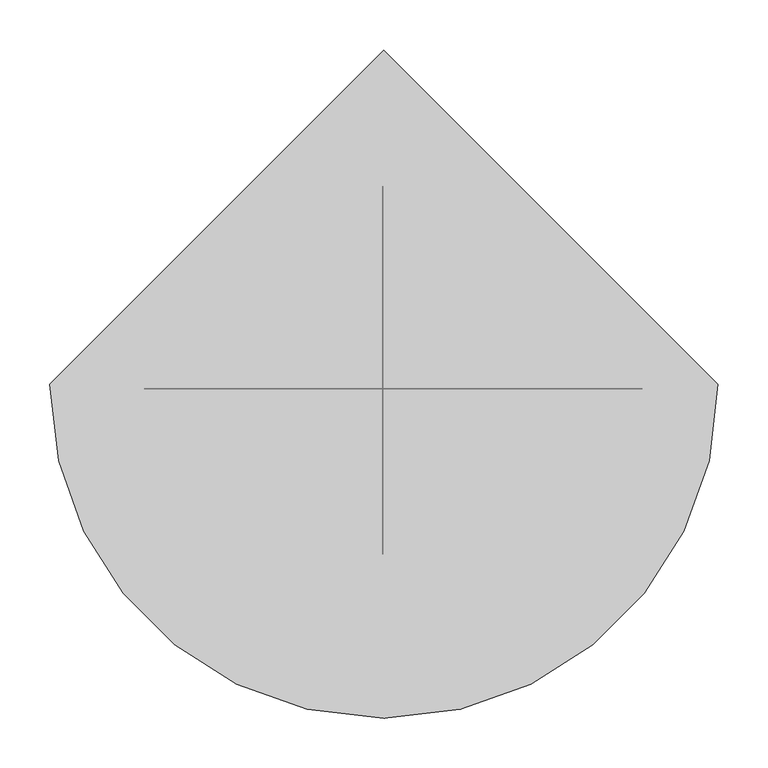
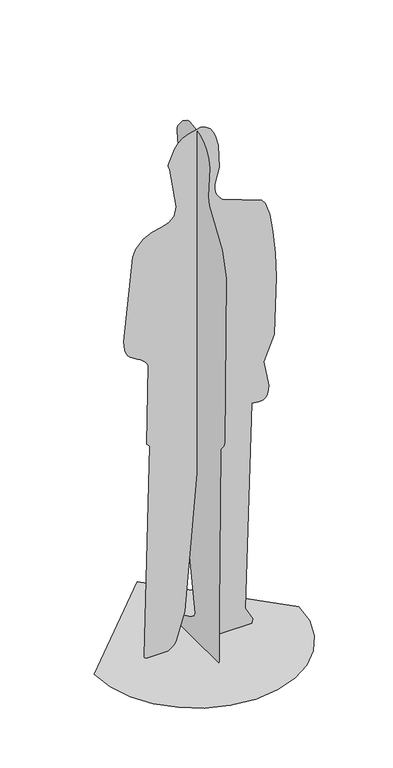
"""IFC4 building model written with IfcOpenShell, lengths in millimetres: proxy geometry, dwayne 23733 : dwayne 23733."""

import ifcopenshell
import ifcopenshell.guid

model = None  # the IFC model being written
_history = None  # IfcOwnerHistory: only IFC2X3 demands one
_inside = {}  # id of a spatial element -> (the spatial element, [elements in it])
_under = {}  # id of a project, library or spatial element -> (it, [spatial elements below it])
_declared = {}  # id of a project -> (the project, [libraries it declares])
_typed = {}  # id of a type object -> (the type object, [elements of that type])
_made_of = {}  # id of a material, layer set ... -> (it, [elements and type objects made of it])


def new_model(schema):
    """Start an empty IFC model of exactly this schema.

    Asked for "IFC4X3", IfcOpenShell would pick the latest addendum, in which some entities
    have other attributes; the version numbers below select the first issue.
    IFC2X3 requires an IfcOwnerHistory on every rooted entity: one is made here for all.
    """
    global model, _history
    if schema == "IFC4X3":
        model = ifcopenshell.file(schema_version=(4, 3, 0, 0))
    else:
        model = ifcopenshell.file(schema=schema)
    _inside.clear()
    _under.clear()
    _declared.clear()
    _typed.clear()
    _made_of.clear()
    _history = None
    if model.schema == "IFC2X3":
        org = make("IfcOrganization", Name="unknown")
        user = make(
            "IfcPersonAndOrganization",
            ThePerson=make("IfcPerson", FamilyName="unknown"),
            TheOrganization=org,
        )
        app = make(
            "IfcApplication",
            ApplicationDeveloper=org,
            Version="unknown",
            ApplicationFullName="unknown",
            ApplicationIdentifier="unknown",
        )
        _history = make(
            "IfcOwnerHistory",
            OwningUser=user,
            OwningApplication=app,
            ChangeAction="ADDED",
            CreationDate=0,
        )
    return model


def make(cls, **values):
    """One entity of the class cls with the attributes given. An attribute that is None is left unset."""
    return model.create_entity(
        cls, **{name: value for name, value in values.items() if value is not None}
    )


def rooted(cls, **values):
    """An entity with a GlobalId (a new one), such as an element, a storey or a relation."""
    return make(cls, GlobalId=ifcopenshell.guid.new(), OwnerHistory=_history, **values)


def si_unit(unit_type, name, prefix=None):
    """IfcSIUnit, for example si_unit("LENGTHUNIT", "METRE", prefix="MILLI")."""
    return make("IfcSIUnit", UnitType=unit_type, Prefix=prefix, Name=name)


def assignment(units):
    """IfcUnitAssignment: the units of a project."""
    return None if units is None else make("IfcUnitAssignment", Units=units)


def point(xyz):
    """IfcCartesianPoint."""
    return None if xyz is None else make("IfcCartesianPoint", Coordinates=xyz)


def direction(xyz):
    """IfcDirection."""
    return None if xyz is None else make("IfcDirection", DirectionRatios=xyz)


def frame(location, z_axis=None, x_axis=None):
    """IfcAxis2Placement3D, a coordinate frame: its origin and axes. An axis left out is left unset."""
    return make(
        "IfcAxis2Placement3D",
        Location=point(location),
        Axis=direction(z_axis),
        RefDirection=direction(x_axis),
    )


def origin():
    """The frame at (0, 0, 0) with its axes left unset."""
    return frame((0.0, 0.0, 0.0))


def place(relative_to, where):
    """IfcLocalPlacement: puts the frame where relative to a parent placement (None: the world)."""
    return make(
        "IfcLocalPlacement", PlacementRelTo=relative_to, RelativePlacement=where
    )


def context(
    kind, dimensions, precision=None, world=None, true_north=None, identifier=None
):
    """IfcGeometricRepresentationContext, for example the 3D "Model" context."""
    return make(
        "IfcGeometricRepresentationContext",
        ContextIdentifier=identifier,
        ContextType=kind,
        CoordinateSpaceDimension=dimensions,
        Precision=precision,
        WorldCoordinateSystem=world,
        TrueNorth=true_north,
    )


def project(units=None, contexts=None):
    """IfcProject with its units and contexts."""
    return rooted(
        "IfcProject",
        Name="project",
        RepresentationContexts=contexts,
        UnitsInContext=assignment(units),
    )


def spatial(cls, under=None, at=None, **own):
    """A site, building, storey or space (cls), placed at a placement, below another one or the project."""
    s = rooted(cls, ObjectPlacement=at, **own)
    if under is not None:
        _under.setdefault(under.id(), (under, []))[1].append(s)
    return s


def point_list(points):
    """IfcCartesianPointList2D or 3D."""
    cls = (
        "IfcCartesianPointList2D" if len(points[0]) == 2 else "IfcCartesianPointList3D"
    )
    return make(cls, CoordList=points)


def triangles(points, corners, closed=None, point_numbers=None):
    """IfcTriangulatedFaceSet: each triangle names its three corners, points numbered from 1."""
    return make(
        "IfcTriangulatedFaceSet",
        Coordinates=point_list(points),
        Closed=closed,
        CoordIndex=corners,
        PnIndex=point_numbers,
    )


def shape(context_of_items, identifier, shape_type, items):
    """IfcShapeRepresentation: the items that make up one representation, for example the "Body"."""
    return make(
        "IfcShapeRepresentation",
        ContextOfItems=context_of_items,
        RepresentationIdentifier=identifier,
        RepresentationType=shape_type,
        Items=items,
    )


def source(mapping_origin, context_of_items, identifier, shape_type, items):
    """IfcRepresentationMap: a shape defined once, which mapped items show again and again."""
    return make(
        "IfcRepresentationMap",
        MappingOrigin=mapping_origin,
        MappedRepresentation=shape(context_of_items, identifier, shape_type, items),
    )


def transform(
    local_origin,
    x_axis=None,
    y_axis=None,
    z_axis=None,
    scale=None,
    scale2=None,
    scale3=None,
    uniform=True,
):
    """IfcCartesianTransformationOperator3D, or its non-uniform kind. x_axis, y_axis, z_axis: its Axis1, 2, 3."""
    if uniform:
        return make(
            "IfcCartesianTransformationOperator3D",
            Axis1=direction(x_axis),
            Axis2=direction(y_axis),
            LocalOrigin=point(local_origin),
            Scale=scale,
            Axis3=direction(z_axis),
        )
    return make(
        "IfcCartesianTransformationOperator3DnonUniform",
        Axis1=direction(x_axis),
        Axis2=direction(y_axis),
        LocalOrigin=point(local_origin),
        Scale=scale,
        Axis3=direction(z_axis),
        Scale2=scale2,
        Scale3=scale3,
    )


def mapped(mapping_source, mapping_target):
    """IfcMappedItem: shows the shape of a source again, moved by a transform."""
    return make(
        "IfcMappedItem", MappingSource=mapping_source, MappingTarget=mapping_target
    )


def made_of(thing, what):
    """Note that an element or type object is made of a material, layer set ...; save() writes the relation."""
    if what is not None:
        _made_of.setdefault(what.id(), (what, []))[1].append(thing)
    return thing


def element(
    cls,
    number,
    at=None,
    inside=None,
    cuts=None,
    type_object=None,
    material=None,
    context=None,
    identifier="Body",
    shape_type=None,
    held_by="IfcProductDefinitionShape",
    body=None,
    shapes=None,
    **own,
):
    """One element of the class cls, such as IfcWall. Its Tag is "e" and its number.

    at: its placement. inside: the storey or other place that contains it. cuts: it is an
    opening in that element (IfcRelVoidsElement). A single representation is given by context,
    identifier, shape_type and body (its items); several are given by shapes. held_by: the class
    of the entity that holds the representations. save() writes the other relations.
    """
    e = rooted(cls, Tag="e%d" % number, ObjectPlacement=at, **own)
    if body is not None:
        shapes = [shape(context, identifier, shape_type, body)]
    if shapes is not None:
        e.Representation = make(held_by, Representations=shapes)
    if inside is not None:
        _inside.setdefault(inside.id(), (inside, []))[1].append(e)
    if cuts is not None:
        rooted(
            "IfcRelVoidsElement", RelatingBuildingElement=cuts, RelatedOpeningElement=e
        )
    if type_object is not None:
        _typed.setdefault(type_object.id(), (type_object, []))[1].append(e)
    return made_of(e, material)


def aggregate(whole, parts):
    """IfcRelAggregates: a whole, such as a stair, and the parts it consists of."""
    return rooted("IfcRelAggregates", RelatingObject=whole, RelatedObjects=parts)


def save(model, path):
    """Write the relations noted so far, then the file.

    IfcRelAggregates (storeys below a building ...), IfcRelContainedInSpatialStructure (elements
    in a storey), IfcRelDefinesByType, IfcRelAssociatesMaterial and IfcRelDeclares: one each for
    every whole, place, type object, material and project.
    """
    for whole, parts in _under.values():
        aggregate(whole, parts)
    for where, things in _inside.values():
        rooted(
            "IfcRelContainedInSpatialStructure",
            RelatedElements=things,
            RelatingStructure=where,
        )
    for kind, things in _typed.values():
        rooted("IfcRelDefinesByType", RelatedObjects=things, RelatingType=kind)
    for what, things in _made_of.values():
        rooted("IfcRelAssociatesMaterial", RelatedObjects=things, RelatingMaterial=what)
    for by, libraries in _declared.values():
        rooted("IfcRelDeclares", RelatingContext=by, RelatedDefinitions=libraries)
    model.write(path)


def entourage_8da15c99(model_context):
    return source(origin(), model_context, "Body", "Tessellation", [
        triangles([(-180.7520848, -4.45e-05, 5.61e-05), (-184.2428783, -8.8e-06, 2.7953159), (-186.1722845, 1.66e-05, 5.8375037), (-186.8317464, 3.35e-05, 9.1275741), (-168.2847317, 8.5e-06, 733.0655743), (-173.8813923, 8.5e-06, 735.2245268), (-177.6699692, 8.1e-06, 740.933626), (-174.1986513, -8.1e-06, 1013.6688681), (-179.5913999, -8.8e-06, 1024.1657564), (-188.0396306, -9.6e-06, 1032.776568), (-198.5268356, -9.9e-06, 1040.1131842), (-210.0364347, -1.03e-05, 1046.7870501), (-221.5521744, -1.07e-05, 1053.4099016), (-232.0573471, -1.1e-05, 1060.5935474), (-240.5355178, -1.14e-05, 1068.9495054), (-245.9520113, -1.21e-05, 1078.9886456), (-249.7388442, -1.29e-05, 1091.9828379), (-252.1553936, -1.4e-05, 1106.9305447), (-253.4609098, -1.47e-05, 1122.8302282), (-224.2189811, -3.16e-05, 1405.0555161), (-213.7950534, -3.31e-05, 1430.2028183), (-189.1320784, -3.46e-05, 1456.0851048), (-160.6250248, -3.53e-05, 1468.8744404), (-131.9230613, -3.57e-05, 1475.6387077), (-106.6753564, -3.64e-05, 1483.4444813), (-88.5310787, -3.71e-05, 1499.3602249), (-81.1393152, -3.9e-05, 1530.4525131), (-102.9420995, -4.71e-05, 1666.4706642), (-107.9473082, -4.78e-05, 1679.2661041), (-108.147514, -4.82e-05, 1680.5750359), (-107.9848786, -4.82e-05, 1682.7597862), (-107.5268942, -4.82e-05, 1685.5199375), (-106.8410076, -4.86e-05, 1688.5562347), (-86.6409597, -5.11e-05, 1733.0913071), (-74.2774747, -5.19e-05, 1747.7193386), (-59.5121968, -5.26e-05, 1759.6604702), (-42.3631437, -5.33e-05, 1768.778809), (-0.985526, -5.37e-05, 1778.0000484), (15.8808848, -5.33e-05, 1772.5538692), (29.1619713, -5.26e-05, 1761.5650051), (39.2640596, -5.19e-05, 1747.0972836), (46.5934905, -5.08e-05, 1731.2151134), (56.0091948, -4.89e-05, 1695.7216404), (59.1639804, -4.41e-05, 1618.2096565), (44.4858611, -4.12e-05, 1564.728764), (44.3096955, -4.05e-05, 1551.1871487), (46.5533085, -3.94e-05, 1537.928801), (51.2886617, -3.86e-05, 1525.4368309), (58.5876893, -3.83e-05, 1514.1934765), (68.5223573, -3.75e-05, 1504.6817024), (198.4031332, -3.46e-05, 1454.5817081), (210.7096676, -3.38e-05, 1440.8303673), (224.9007164, -3.13e-05, 1397.8456364), (235.5370584, -2.72e-05, 1333.6076969), (242.7581838, -2.28e-05, 1256.1539944), (246.7033826, -1.77e-05, 1173.5217562), (240.2782843, -5.9e-06, 974.9295902), (206.0815162, -1.1e-06, 891.6227566), (221.1963095, 4e-06, 805.6638319), (220.4651949, 5.1e-06, 788.6204681), (214.9949983, 6.3e-06, 771.8049974), (210.3553288, 6.6e-06, 765.7305136), (204.1669347, 6.6e-06, 762.0923635), (196.896103, 7e-06, 760.3986443), (189.0091026, 7e-06, 760.1578159), (180.9722385, 7e-06, 760.8779028), (173.2516706, 6.6e-06, 762.0673651), (166.3136674, 6.6e-06, 763.2343723), (144.8011997, 4.49e-05, 59.4753214), (168.6276432, 4.74e-05, 15.3365923), (166.1986854, -4.45e-05, 5.61e-05), (66.1332453, -4.45e-05, 5.61e-05), (49.8425291, -1.03e-05, 3.9765614), (39.0246438, 1.36e-05, 14.0353079), (32.5983191, 2.91e-05, 28.3297275), (-2.744106, 9.2e-06, 720.0463108), (-54.0725352, 1.03e-05, 117.9433913), (-81.3720589, -2.13e-05, 28.0047586), (-85.5237496, -2.69e-05, 19.9172799), (-91.2434313, -3.27e-05, 12.5691251), (-99.2452049, -3.86e-05, 5.9378921), (-110.2432618, -4.45e-05, 5.61e-05), (-13.8237486, -127.6719491, 9.9621213), (-13.8238053, -127.261836, 182.0843436), (-13.8237894, -135.2636459, 744.8700136), (-13.8237894, -136.4150655, 748.3464729), (-13.8237894, -139.3955521, 752.5740492), (-13.8237894, -143.4944844, 757.5063063), (-13.8237894, -148.0011678, 763.0967354), (-13.8237894, -152.2050719, 769.2988277), (-13.8237872, -155.3954567, 776.0660746), (-13.8237872, -156.8617189, 783.3521124), (-13.8237701, -165.9465932, 1358.6144554), (-13.8237679, -143.2744033, 1442.0936623), (-13.8237656, -71.1145909, 1552.8595757), (-13.8237656, -64.3402088, 1580.52155), (-13.8237622, -73.5344423, 1684.7962898), (-13.823761, -67.2131621, 1712.2171452), (-13.823761, -55.2412548, 1734.9080566), (-13.823761, -37.926044, 1752.7547871), (-13.823761, -15.5748862, 1765.6435352), (-13.823761, 11.5049153, 1773.4603546), (-13.823761, 43.0060141, 1776.0911533), (-13.823761, 55.0860544, 1772.9175098), (-13.8237622, 79.7039013, 1756.3228832), (-13.8237633, 107.489678, 1722.3487942), (-13.8237633, 111.5712331, 1713.0111374), (-13.8237633, 112.222992, 1702.3029247), (-13.8237667, 99.0832871, 1611.9293713), (-13.8237667, 100.6007817, 1597.8216568), (-13.8237679, 96.7552315, 1579.0665516), (-13.8237701, 31.1784748, 1488.4601635), (-13.8237815, 125.7984987, 1146.7478817), (-13.8237815, 134.1994394, 1137.675761), (-13.8237826, 184.2800127, 1119.3932287), (-13.8237826, 194.4650741, 1111.9401226), (-13.8237826, 201.1344345, 1100.3807991), (-13.8237849, 203.5509657, 1084.206423), (-13.8237849, 200.9675115, 1068.9646208), (-13.8237849, 194.2821819, 1055.8713066), (-13.8237849, 184.3929236, 1046.1421766), (-13.8237849, 172.1979195, 1040.9932903), (-13.8237849, 158.5950979, 1041.6405619), (-13.8237849, 144.4825418, 1049.2996874), (-13.8237917, 123.0430165, 785.7652645), (-13.8237928, 116.9063816, 707.2433859), (-13.8238008, 10.2023739, 90.6853713), (-13.8238019, 17.9839052, 76.1482317), (-13.8238031, 35.4714609, 63.8067794), (-13.8238121, 104.5965861, 31.8661645), (-13.8238133, 119.3345128, 20.2173774), (-13.8238155, 122.9915752, 6.7192125), (-13.8238121, 122.0607817, 4.3675023), (-13.8237974, 120.3452433, 2.3141491), (-13.8237803, 119.1854304, 1.4285661), (-13.8237542, 117.8200159, 0.6534775), (-13.8237179, 116.2459023, 5.61e-05), (-13.8237156, -124.5016756, 0.0), (-348.4736423, 4.7230064, 0.0001684), (-339.5989297, -72.1961928, 0.0001684), (-314.3239463, -142.8341776, 5.61e-05), (-274.6723876, -205.1670917, 5.61e-05), (-222.6682945, -257.1712393, 5.61e-05), (-160.3353441, -296.8226708, 5.61e-05), (-89.6973684, -322.0977087, 5.61e-05), (-12.7781717, -330.9724577, 5.61e-05), (64.1410249, -322.097745, 5.61e-05), (134.7790189, -296.8227253, 5.61e-05), (197.1119329, -257.171203, 5.61e-05), (249.1161351, -205.167128, 5.61e-05), (288.7675302, -142.8341413, 5.61e-05), (314.0425681, -72.1961383, 0.0001684), (322.9173171, 4.7230359, 0.0001684), (-12.7782308, 340.4184654, 0.0001684)], [[70, 71, 72], [69, 70, 72], [69, 72, 73], [69, 73, 74], [69, 74, 75], [69, 75, 76], [68, 69, 76], [82, 1, 2], [82, 2, 3], [82, 3, 4], [81, 82, 4], [80, 81, 4], [79, 80, 4], [78, 79, 4], [77, 78, 4], [77, 4, 5], [76, 77, 5], [5, 6, 7], [76, 5, 7], [76, 7, 8], [68, 76, 8], [67, 68, 8], [66, 67, 8], [65, 66, 8], [64, 65, 8], [63, 64, 8], [62, 63, 8], [61, 62, 8], [60, 61, 8], [59, 60, 8], [58, 59, 8], [57, 58, 8], [56, 57, 8], [56, 8, 9], [55, 56, 9], [55, 9, 10], [54, 55, 10], [54, 10, 11], [53, 54, 11], [53, 11, 12], [52, 53, 12], [51, 52, 12], [50, 51, 12], [50, 12, 13], [50, 13, 14], [50, 14, 15], [50, 15, 16], [50, 16, 17], [50, 17, 18], [50, 18, 19], [50, 19, 20], [50, 20, 21], [50, 21, 22], [50, 22, 23], [50, 23, 24], [50, 24, 25], [50, 25, 26], [49, 50, 26], [48, 49, 26], [48, 26, 27], [47, 48, 27], [46, 47, 27], [45, 46, 27], [44, 45, 27], [44, 27, 28], [43, 44, 28], [42, 43, 28], [42, 28, 29], [42, 29, 30], [42, 30, 31], [42, 31, 32], [42, 32, 33], [42, 33, 34], [42, 34, 35], [42, 35, 36], [42, 36, 37], [41, 42, 37], [40, 41, 37], [40, 37, 38], [40, 38, 39], [137, 138, 83], [137, 83, 84], [136, 137, 84], [135, 136, 84], [130, 131, 132], [130, 132, 133], [130, 133, 134], [130, 134, 135], [122, 123, 124], [121, 122, 124], [120, 121, 124], [119, 120, 124], [118, 119, 124], [117, 118, 124], [116, 117, 124], [115, 116, 124], [114, 115, 124], [113, 114, 124], [106, 107, 108], [105, 106, 108], [104, 105, 108], [103, 104, 108], [102, 103, 108], [101, 102, 108], [100, 101, 108], [99, 100, 108], [98, 99, 108], [97, 98, 108], [97, 108, 109], [97, 109, 110], [97, 110, 111], [96, 97, 111], [95, 96, 111], [95, 111, 112], [94, 95, 112], [93, 94, 112], [93, 112, 113], [92, 93, 113], [92, 113, 124], [92, 124, 125], [91, 92, 125], [90, 91, 125], [89, 90, 125], [88, 89, 125], [87, 88, 125], [86, 87, 125], [86, 125, 126], [85, 86, 126], [85, 126, 127], [84, 85, 127], [84, 127, 128], [135, 84, 128], [135, 128, 129], [130, 135, 129], [153, 154, 139], [152, 153, 139], [152, 139, 140], [151, 152, 140], [151, 140, 141], [151, 141, 142], [150, 151, 142], [149, 150, 142], [149, 142, 143], [149, 143, 144], [149, 144, 145], [149, 145, 146], [149, 146, 147], [149, 147, 148]], closed=False),
    ])


if __name__ == "__main__":
    model = new_model("IFC4")
    model_context = context("Model", 3, world=origin())
    ifc_project = project(units=[si_unit("LENGTHUNIT", "METRE", prefix="MILLI")], contexts=[model_context])
    site = spatial("IfcSite", under=ifc_project)
    building = spatial("IfcBuilding", under=site)
    placement = place(None, origin())
    entourage_shape = entourage_8da15c99(model_context)
    element("IfcBuildingElementProxy", 1, Name="dwayne 23733 : dwayne 23733", ObjectType="dwayne 23733 : dwayne 23733", at=placement, inside=building, context=model_context, shape_type="MappedRepresentation", body=[
        mapped(entourage_shape, transform((0.0, 0.0, 0.0), x_axis=(1.0, 0.0, 0.0), y_axis=(0.0, 1.0, 0.0), z_axis=(0.0, 0.0, 1.0))),
    ])
    save(model, "model.ifc")

# Revit data of these elements
# Type "dwayne 23733 : dwayne 23733"
#   built-in parameter 1005195 = "RPC-8-G1AE-S4G0-CKUK-A"
#   Height = 0
